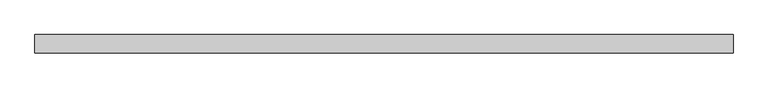
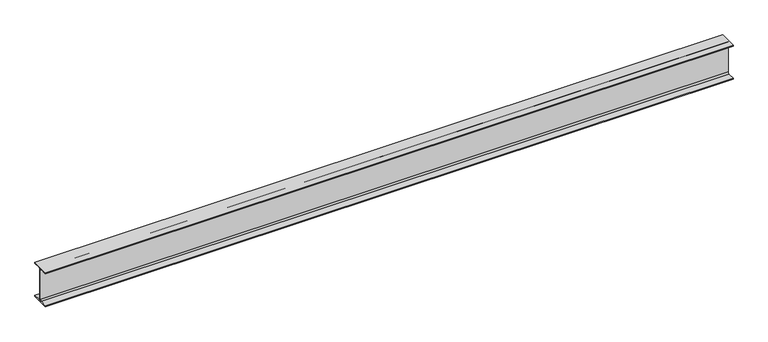
"""IFC4 building model written with IfcOpenShell, lengths in millimetres: beam geometry, 0912_Steel Framing_H-KSD3502 : H_SB_ASB_H-350x175x7x11."""

from ifc_helpers import new_model, si_unit, point, frame, frame_2d, origin, place, context, project, spatial, polyline, circle_curve, trimmed, segment, composite_curve, outline, extrude, source, transform, mapped, element, save


def beam_3a100c14(model_context):
    return source(origin(), model_context, "Body", "SweptSolid", [
        extrude(outline(composite_curve([segment(polyline([(87.5, -164.0), (87.5, -175.0), (-87.5, -175.0), (-87.5, -164.0), (-17.5, -164.0)]), True, "CONTINUOUS"), segment(trimmed(circle_curve(frame_2d((-17.5, -150.0)), 14.0), [point((-17.5, -164.0))], [point((-3.5, -150.0))], True, "CARTESIAN"), True, "CONTINUOUS"), segment(polyline([(-3.5, -150.0), (-3.5, 150.0)]), True, "CONTINUOUS"), segment(trimmed(circle_curve(frame_2d((-17.5, 150.0)), 14.0), [point((-3.5, 150.0))], [point((-17.5, 164.0))], True, "CARTESIAN"), True, "CONTINUOUS"), segment(polyline([(-17.5, 164.0), (-87.5, 164.0), (-87.5, 175.0), (87.5, 175.0), (87.5, 164.0), (17.5, 164.0)]), True, "CONTINUOUS"), segment(trimmed(circle_curve(frame_2d((17.5, 150.0)), 14.0), [point((17.5, 164.0))], [point((3.5, 150.0))], True, "CARTESIAN"), True, "CONTINUOUS"), segment(polyline([(3.5, 150.0), (3.5, -150.0)]), True, "CONTINUOUS"), segment(trimmed(circle_curve(frame_2d((17.5, -150.0)), 14.0), [point((3.5, -150.0))], [point((17.5, -164.0))], True, "CARTESIAN"), True, "CONTINUOUS"), segment(polyline([(17.5, -164.0), (87.5, -164.0)]), True, "CONTINUOUS")], self_intersect=False)), frame((-3337.3, 0.0, 0.0), z_axis=(1.0, 0.0, 0.0), x_axis=(0.0, 1.0, 0.0)), (0.0, 0.0, 1.0), 6674.6),
    ])


if __name__ == "__main__":
    model = new_model("IFC4")
    model_context = context("Model", 3, world=origin())
    ifc_project = project(units=[si_unit("LENGTHUNIT", "METRE", prefix="MILLI")], contexts=[model_context])
    site = spatial("IfcSite", under=ifc_project)
    building = spatial("IfcBuilding", under=site)
    placement = place(None, origin())
    beam_shape = beam_3a100c14(model_context)
    element("IfcBeam", 1, ObjectType="0912_Steel Framing_H-KSD3502 : H_SB_ASB_H-350x175x7x11", at=placement, inside=building, context=model_context, shape_type="MappedRepresentation", body=[
        mapped(beam_shape, transform((0.0, 0.0, 0.0), x_axis=(1.0, 0.0, 0.0), y_axis=(0.0, 1.0, 0.0), z_axis=(0.0, 0.0, 1.0))),
    ])
    save(model, "model.ifc")

# Revit data of these elements
# Type "0912_Steel Framing_H-KSD3502 : H_SB_ASB_H-350x175x7x11"
#   H_WM Code_1 = "S01AA002-00001 | Main Steel Structure Fabrication Work | Shelter/Building | Medium Steel - Standard (90KG/M>Weight≥30KG/M) | Material: (   )"
#   H_WM Code_2 = "S03AA028-00001 | Main Steel Structure Erection Work | Shelter/Building | Medium Steel (90KG/M>Weight≥30KG/M) | Material: (   )"
#   H_WM Code_3 = "S01AA010-00001 | Main Steel Structure Fabrication Work | Shelter/Building | Steel Painting/Coating | for Non-Fireproofed Steel Surface, Surface Preparation, Primer, Second & Final Coat | Material: (   )"
#   H_Q'ty Cal Type Tag = "SB-Q2"
#   Width = 17.5 cm
#   Web Thickness = 0.7 cm
#   Web Fillet = 1.4 cm
#   Warping Constant = 282000.0 cm⁶
#   W = 0
#   Torsional Moment of Inertia = 19.4042 cm⁴
#   Section Area = 63.14 cm²
#   Plastic Modulus weak axis = 174.0 cm³
#   Plastic Modulus strong axis = 868.0 cm³
#   Perimeter = 1.36 m²/m
#   Nominal Weight = 49.60 kgf/m
#   Moment of Inertia weak axis = 984.00 cm⁴
#   Moment of Inertia strong axis = 13600.00 cm⁴
#   Height = 35.0 cm
#   Flange Thickness = 1.1 cm
#   Elastic Modulus weak axis = 112.0 cm³
#   Elastic Modulus strong axis = 775.0 cm³
#   Centroid Vertical = 17.5 cm
#   Centroid Horizontal = 8.75 cm
#   Ix = 136000000
#   Length [instance default] = 1.5240 m
#   Zx = 868000
#   b = 0.1750 m
#   h = 0.3500 m
#   r = 0.0140 m
#   s = 0.0070 m
#   t = 0.0110 m
#   A = 0.006314 m²
#   Structural Material [instance default] = Steel, 45-345
#   Assembly Code = ""
# Element 1 (IfcBeam, "0912_Steel Framing_H-KSD3502 : H_SB_ASB_H-350x175x7x11")
#   Structural Material = none
# Materials
#   "Steel, 45-345": class "Metal", colour RGB 189 187 185, transparency 0, Description = "Steel 345 MPa", Cost = 0
